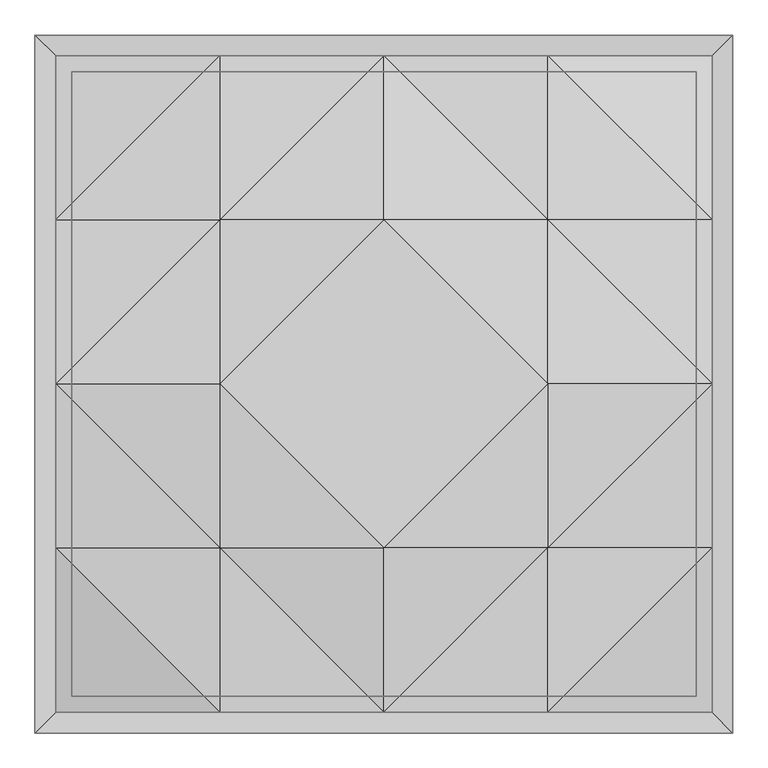
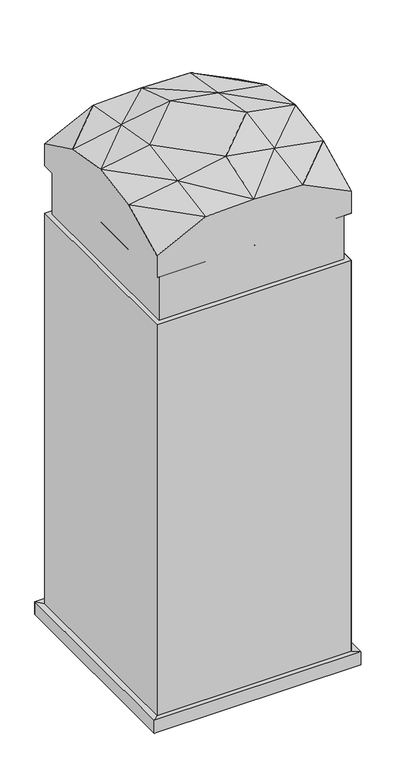
"""IFC4 building model written with IfcOpenShell, lengths in millimetres: geographic element geometry, Enscape AssetDefinition - Phonebooth 001 : Enscape AssetDefinition - Phonebooth 001."""

from ifc_helpers import new_model, si_unit, origin, place, context, project, spatial, triangles, source, transform, mapped, element, save


def geographic_element_4e0d1d1e(model_context):
    return source(origin(), model_context, "Body", "Tessellation", [
        triangles([(535.4750187, 563.9070405, 65.5929985), (-535.4750187, -563.9070405, 65.5929985), (563.9070405, -563.9070405, 73.6019982), (-530.4179873, -530.4179873, 69.2310031), (-530.4179873, 530.4179873, 2320.0650719), (-563.9070405, -563.9070405, 73.6019982), (-530.4179873, -530.4179873, 2320.0650719), (-504.6510281, -504.6510281, 2320.0650719), (-504.6510281, -504.6510281, 2591.2188698), (-504.6510281, 504.6510281, 2320.0650719), (504.6510281, 504.6510281, 2320.0650719), (530.4179873, 530.4179873, 2320.0650719), (504.6510281, -504.6510281, 2320.0650719), (504.6510281, 504.6510281, 2591.2188698), (-530.4179873, 530.4179873, 69.2310031), (530.4179873, -530.4179873, 2320.0650719), (530.4179873, -530.4179873, 69.2310031), (530.4179873, 530.4179873, 69.2310031), (-563.9070405, 563.9070405, 73.6019982), (563.9070405, 563.9070405, 0.0), (-535.4750187, 563.9070405, 65.5929985), (-563.9070405, 563.9070405, 0.0), (-563.9070405, -563.9070405, 0.0), (535.4750187, -563.9070405, 65.5929985), (563.9070405, -563.9070405, 0.0), (563.9070405, 563.9070405, 73.6019982), (-530.4179873, 0.0, 2591.2188698), (0.0, -530.4179873, 2591.2188698), (530.4179873, -530.4179873, 2591.2188698), (504.6510281, -504.6510281, 2591.2188698), (0.0, 530.4179873, 2591.2188698), (-504.6510281, 504.6510281, 2591.2188698), (-265.2089936, 530.4179873, 2848.6720505), (530.4179873, 530.4179873, 2591.2188698), (265.2089936, 530.4179873, 2848.6720505), (530.4179873, 530.4179873, 2717.9288681), (530.4179873, 265.2089936, 2848.6720505), (0.0, 265.2089936, 2942.3451118), (0.0, 530.4179873, 2855.5079704), (-265.2089936, 265.2089936, 2895.5090172), (265.2089936, 0.0, 2942.3451118), (265.2089936, 265.2089936, 2895.5090172), (530.4179873, 0.0, 2892.5769287), (265.2089936, -265.2089936, 2895.5090172), (0.0, 0.0, 2942.3451118), (-265.2089936, 0.0, 2942.3451118), (0.0, -265.2089936, 2942.3451118), (0.0, -530.4179873, 2855.5079704), (-530.4179873, -265.2089936, 2848.6720505), (-265.2089936, -265.2089936, 2895.5090172), (-530.4179873, 0.0, 2892.5769287), (-530.4179873, 265.2089936, 2848.6720505), (-530.4179873, -530.4179873, 2717.9288681), (-530.4179873, -530.4179873, 2591.2188698), (-265.2089936, -530.4179873, 2848.6720505), (265.2089936, -530.4179873, 2848.6720505), (530.4179873, -265.2089936, 2848.6720505), (530.4179873, -530.4179873, 2717.9288681), (530.4179873, 0.0, 2591.2188698), (-530.4179873, 530.4179873, 2591.2188698), (-530.4179873, 530.4179873, 2717.9288681)], [[33, 52, 40], [33, 61, 52], [60, 61, 33], [60, 52, 61], [60, 27, 52], [57, 56, 58], [29, 59, 57], [29, 58, 56], [29, 57, 58], [29, 56, 28], [54, 28, 55], [54, 55, 53], [49, 53, 55], [54, 53, 49], [54, 49, 27], [40, 52, 51], [27, 49, 51], [27, 51, 52], [40, 51, 46], [51, 49, 50], [51, 50, 46], [49, 55, 50], [50, 55, 48], [28, 56, 48], [28, 48, 55], [57, 44, 56], [44, 48, 56], [46, 50, 47], [44, 47, 48], [50, 48, 47], [46, 47, 45], [38, 40, 46], [38, 46, 45], [41, 45, 47], [38, 45, 41], [41, 47, 44], [43, 41, 44], [43, 44, 57], [59, 43, 57], [59, 37, 43], [42, 41, 43], [42, 43, 37], [38, 41, 42], [39, 38, 42], [39, 33, 40], [39, 40, 38], [35, 42, 37], [39, 42, 35], [35, 37, 36], [34, 36, 37], [34, 35, 36], [34, 37, 59], [34, 31, 35], [31, 33, 39], [31, 39, 35], [60, 33, 31], [27, 60, 32], [32, 60, 31], [14, 34, 59], [31, 34, 14], [31, 14, 32], [59, 29, 30], [30, 29, 28], [59, 30, 14], [9, 54, 27], [28, 54, 9], [27, 32, 9], [28, 9, 30], [26, 1, 21], [26, 25, 20], [26, 3, 25], [26, 17, 3], [3, 23, 25], [6, 2, 24], [3, 6, 23], [6, 24, 3], [6, 22, 23], [6, 19, 22], [19, 26, 20], [26, 21, 19], [19, 20, 22], [6, 15, 19], [26, 18, 17], [19, 15, 18], [19, 18, 26], [18, 16, 17], [15, 5, 12], [18, 12, 16], [15, 12, 18], [13, 30, 9], [16, 12, 13], [11, 14, 30], [12, 11, 13], [11, 30, 13], [10, 32, 14], [12, 5, 10], [10, 14, 11], [12, 10, 11], [8, 9, 32], [16, 13, 8], [8, 32, 10], [13, 9, 8], [7, 8, 10], [5, 7, 10], [16, 8, 7], [4, 17, 16], [6, 4, 15], [3, 17, 4], [4, 7, 5], [4, 16, 7], [3, 4, 6], [4, 5, 15]], closed=False),
    ])


if __name__ == "__main__":
    model = new_model("IFC4")
    model_context = context("Model", 3, world=origin())
    ifc_project = project(units=[si_unit("LENGTHUNIT", "METRE", prefix="MILLI")], contexts=[model_context])
    site = spatial("IfcSite", under=ifc_project)
    building = spatial("IfcBuilding", under=site)
    placement = place(None, origin())
    geographic_element_shape = geographic_element_4e0d1d1e(model_context)
    element("IfcGeographicElement", 1, ObjectType="Enscape AssetDefinition - Phonebooth 001 : Enscape AssetDefinition - Phonebooth 001", at=placement, inside=building, context=model_context, shape_type="MappedRepresentation", body=[
        mapped(geographic_element_shape, transform((0.0, 0.0, 0.0), x_axis=(1.0, 0.0, 0.0), y_axis=(0.0, 1.0, 0.0), z_axis=(0.0, 0.0, 1.0))),
    ])
    save(model, "model.ifc")

# Revit data of these elements
# Type "Enscape AssetDefinition - Phonebooth 001 : Enscape AssetDefinition - Phonebooth 001"
#   EnscapeAssetSource = "REMOTE"
#   EnscapeAssetId = "cbaa4123-c8af-4927-a697-0b826d016a1a"
#   Height = 2.942345 m
#   EnscapeNativeAssetHeight = 2.942345 m
#   Default Elevation = 0
